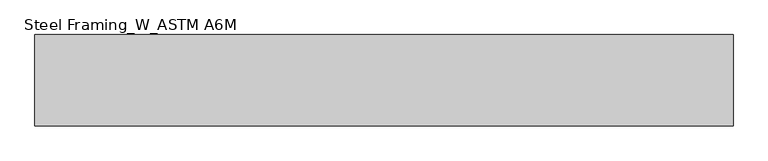
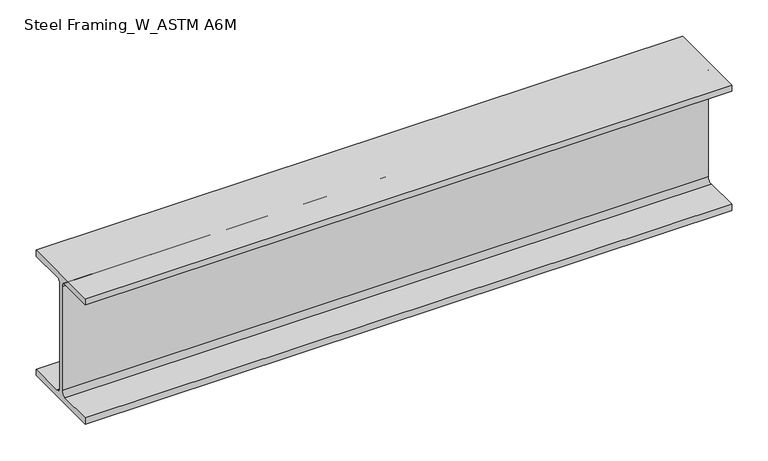
"""IFC4 building model written with IfcOpenShell, lengths in millimetres: beam geometry, Steel Framing_W_ASTM A6M : H_SB_AR_S02_W200x31.3_B6."""

from ifc_helpers import new_model, si_unit, point, frame, frame_2d, origin, place, context, project, spatial, polyline, circle_curve, trimmed, segment, composite_curve, outline, extrude, source, transform, mapped, element, save


def steel_framing_w_astm_a6m_a4340d73(model_context):
    return source(origin(), model_context, "Body", "SweptSolid", [
        extrude(outline(composite_curve([segment(polyline([(67.0, -94.8), (67.0, -105.0), (-67.0, -105.0), (-67.0, -94.8), (-10.775, -94.8)]), True, "CONTINUOUS"), segment(trimmed(circle_curve(frame_2d((-10.775, -87.2)), 7.6), [point((-10.775, -94.8))], [point((-3.175, -87.2))], True, "CARTESIAN"), True, "CONTINUOUS"), segment(polyline([(-3.175, -87.2), (-3.175, 87.2)]), True, "CONTINUOUS"), segment(trimmed(circle_curve(frame_2d((-10.775, 87.2)), 7.6), [point((-3.175, 87.2))], [point((-10.775, 94.8))], True, "CARTESIAN"), True, "CONTINUOUS"), segment(polyline([(-10.775, 94.8), (-67.0, 94.8), (-67.0, 105.0), (67.0, 105.0), (67.0, 94.8), (10.775, 94.8)]), True, "CONTINUOUS"), segment(trimmed(circle_curve(frame_2d((10.775, 87.2)), 7.6), [point((10.775, 94.8))], [point((3.175, 87.2))], True, "CARTESIAN"), True, "CONTINUOUS"), segment(polyline([(3.175, 87.2), (3.175, -87.2)]), True, "CONTINUOUS"), segment(trimmed(circle_curve(frame_2d((10.775, -87.2)), 7.6), [point((3.175, -87.2))], [point((10.775, -94.8))], True, "CARTESIAN"), True, "CONTINUOUS"), segment(polyline([(10.775, -94.8), (67.0, -94.8)]), True, "CONTINUOUS")], self_intersect=False)), frame((-511.3, 0.0, 0.0), z_axis=(1.0, 0.0, 0.0), x_axis=(0.0, 1.0, 0.0)), (0.0, 0.0, 1.0), 1022.6),
    ])


if __name__ == "__main__":
    model = new_model("IFC4")
    model_context = context("Model", 3, world=origin())
    ifc_project = project(units=[si_unit("LENGTHUNIT", "METRE", prefix="MILLI")], contexts=[model_context])
    site = spatial("IfcSite", under=ifc_project)
    building = spatial("IfcBuilding", under=site)
    placement = place(None, origin())
    steel_framing_w_astm_a6m_shape = steel_framing_w_astm_a6m_a4340d73(model_context)
    element("IfcBeam", 1, ObjectType="Steel Framing_W_ASTM A6M : H_SB_AR_S02_W200x31.3_B6", at=placement, inside=building, context=model_context, shape_type="MappedRepresentation", body=[
        mapped(steel_framing_w_astm_a6m_shape, transform((0.0, 0.0, 0.0), x_axis=(1.0, 0.0, 0.0), y_axis=(0.0, 1.0, 0.0), z_axis=(0.0, 0.0, 1.0))),
    ])
    save(model, "model.ifc")

# Revit data of these elements
# Type "Steel Framing_W_ASTM A6M : H_SB_AR_S02_W200x31.3_B6"
#   Type Mark = "B6"
#   Section Name Key = "W8x21"
#   Width = 13.4 cm
#   Web Thickness = 0.635 cm
#   Web Fillet = 0.76 cm
#   Warping Constant = 40800.0 cm⁶
#   Torsional Moment of Inertia = 11.70 cm⁴
#   Section Area = 39.7 cm²
#   Plastic Modulus weak axis = 93.2 cm³
#   Plastic Modulus strong axis = 334.0 cm³
#   Perimeter = 0.93 m²/m
#   Nominal Weight = 31.30 kgf/m
#   Moment of Inertia weak axis = 407.00 cm⁴
#   Moment of Inertia strong axis = 3130.00 cm⁴
#   Height = 21.0 cm
#   Flange Thickness = 1.02 cm
#   Elastic Modulus weak axis = 60.8 cm³
#   Elastic Modulus strong axis = 298.0 cm³
#   Centroid Vertical = 10.5 cm
#   Centroid Horizontal = 6.7 cm
#   Length [instance default] = 1500 mm
#   Structural Material [instance default] = Steel, 45-345
#   Bolt Spacing = 0
#   Assembly Code = ""
# Element 1 (IfcBeam, "Steel Framing_W_ASTM A6M : H_SB_AR_S02_W200x31.3_B6")
#   Materials on its faces: "Steel, 45-345"
# Materials
#   "Steel, 45-345": class "Metal", colour RGB 189 187 185, transparency 0, Description = "Steel 345 MPa", Cost = 0
